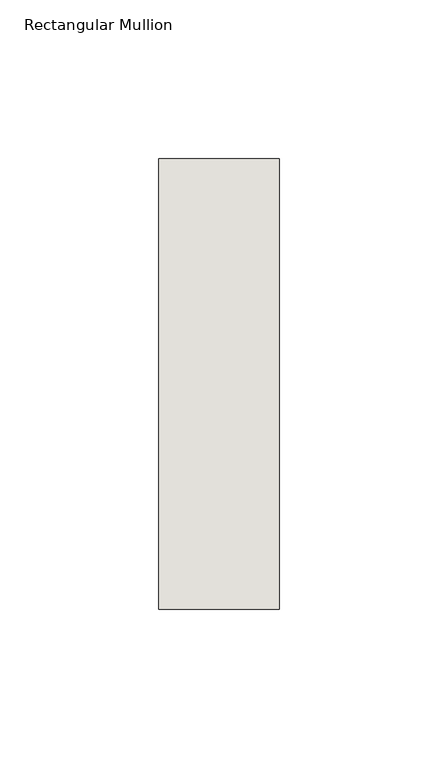
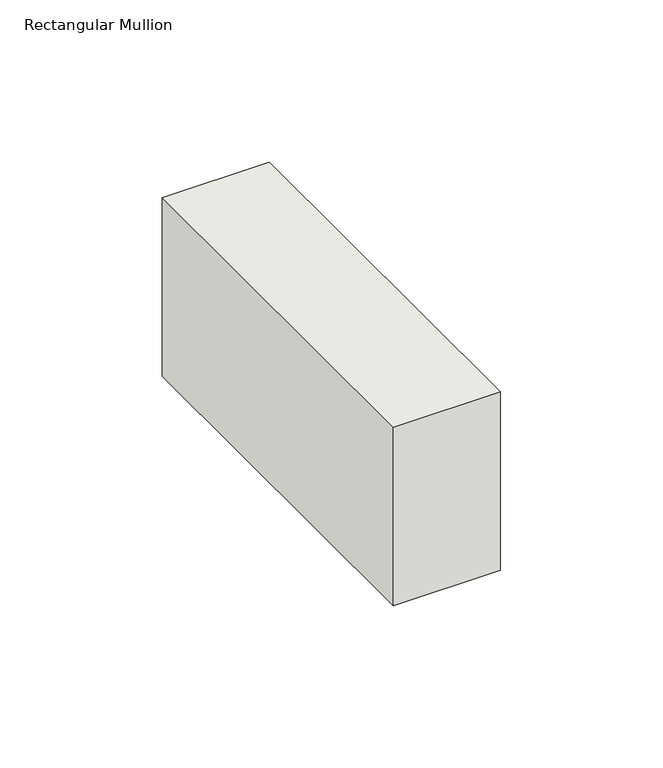
"""IFC4 building model written with IfcOpenShell, lengths in millimetres: wall geometry, Rectangular Mullion : NLRS_21_CWM_hsb-regel 38x142_gen_rsf."""

from ifc_helpers import new_model, si_unit, frame, origin, place, context, project, spatial, polyline, outline, extrude, source, transform, mapped, element, save


def rectangular_mullion_8284db35(model_context):
    return source(origin(), model_context, "Body", "SweptSolid", [
        extrude(outline(polyline([(-38.0, -71.0), (-38.0, 71.0), (0.0, 71.0), (0.0, -71.0), (-38.0, -71.0)])), frame((0.0, 0.0, -66.9999997), z_axis=(0.0, 0.0, 1.0), x_axis=(1.0, 0.0, 0.0)), (0.0, 0.0, 1.0), 66.9999997),
    ])


if __name__ == "__main__":
    model = new_model("IFC4")
    model_context = context("Model", 3, world=origin())
    ifc_project = project(units=[si_unit("LENGTHUNIT", "METRE", prefix="MILLI")], contexts=[model_context])
    site = spatial("IfcSite", under=ifc_project)
    building = spatial("IfcBuilding", under=site)
    placement = place(None, origin())
    rectangular_mullion_shape = rectangular_mullion_8284db35(model_context)
    element("IfcWall", 1, ObjectType="Rectangular Mullion : NLRS_21_CWM_hsb-regel 38x142_gen_rsf", at=placement, inside=building, context=model_context, shape_type="MappedRepresentation", body=[
        mapped(rectangular_mullion_shape, transform((0.0, 0.0, 0.0), x_axis=(1.0, 0.0, 0.0), y_axis=(0.0, 1.0, 0.0), z_axis=(0.0, 0.0, 1.0))),
    ])
    save(model, "model.ifc")

# Revit data of these elements
# Type "Rectangular Mullion : NLRS_21_CWM_hsb-regel 38x142_gen_rsf"
#   Type IfcGUID = "07M7mRoiH1CR8m_RSKIwpF"
#   Assembly Code = "21.10"
#   IfcExportAs = "IfcWall"
#   built-in parameter 1007322 = 0.465879 (stored number, unit not read)
#   built-in parameter 1007321 = 0.062336 (stored number, unit not read)
#   built-in parameter 1007320 = 0.062336 (stored number, unit not read)
# Element 1 (IfcWall, "Rectangular Mullion : NLRS_21_CWM_hsb-regel 38x142_gen_rsf")
#   Materials on its faces: "NLRS_i2_hout naaldhout vuren_gen_rsf"
# Materials
#   "NLRS_i2_hout naaldhout vuren_gen_rsf": class "I - Hout", colour RGB 234 199 147, transparency 0, Keynote = "i2", Manufacturer = "Revit Standards Foundation", URL = "www.revitstandards.org", Description = "hout vuren", Cost = 0
